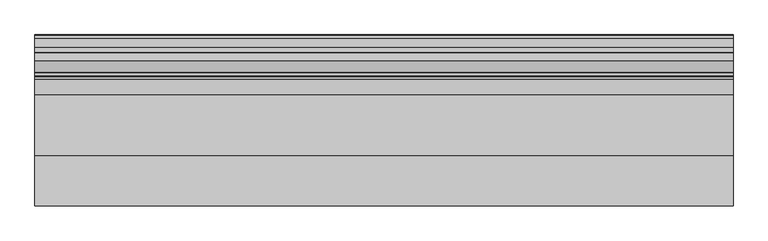
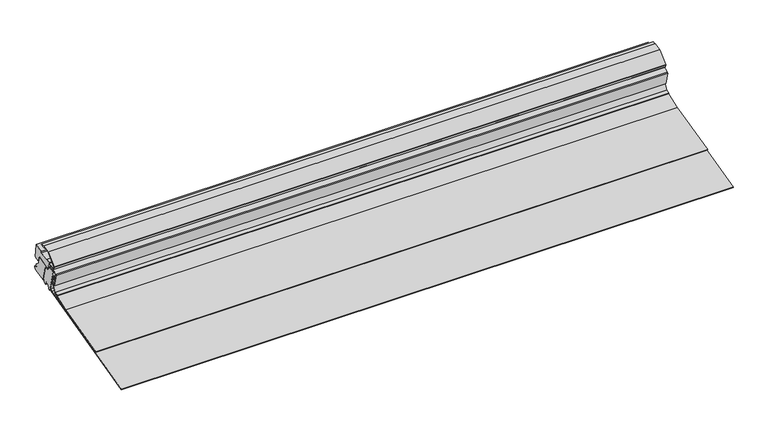
"""IFC4 building model written with IfcOpenShell, lengths in millimetres: proxy geometry, Skylight profile001 901 : Skylight profile001 901."""

from ifc_helpers import new_model, si_unit, frame, origin, place, context, project, spatial, polyline, outline, extrude, source, transform, mapped, element, save


def generic_models_6a062e64(model_context):
    return source(origin(), model_context, "Body", "SweptSolid", [
        extrude(outline(polyline([(9523.9829599, 43669.7464426), (9351.4552326, 43627.7409442), (9350.9821116, 43629.6841777), (9523.3822066, 43671.6586013), (9583.8408702, 43695.1080629), (9584.5640949, 43693.2434059), (9523.9829599, 43669.7464426)])), frame((3694.2883192, 0.0, 0.0), z_axis=(1.0, 0.0, 0.0), x_axis=(0.0, 1.0, 0.0)), (0.0, 0.0, 1.0), 2000.0),
        extrude(outline(polyline([(9598.5792608, 43722.029488), (9582.301634, 43695.3705298), (9570.3578071, 43691.0700225), (9569.6802664, 43692.9517607), (9580.9616075, 43697.0137327), (9596.4357486, 43722.3567685), (9592.5767442, 43737.7822152), (9594.516951, 43738.2675993), (9598.5792608, 43722.029488)])), frame((3694.2883192, 0.0, 0.0), z_axis=(1.0, 0.0, 0.0), x_axis=(0.0, 1.0, 0.0)), (0.0, 0.0, 1.0), 2000.0),
        extrude(outline(polyline([(9608.548635, 43692.8894811), (9604.1362045, 43685.5534517), (9206.9695462, 43585.9015861), (9206.4828193, 43587.8414565), (9602.8481566, 43687.2922651), (9606.4085244, 43693.21167), (9594.4616464, 43741.4763112), (9596.4030551, 43741.9568653), (9608.548635, 43692.8894811)])), frame((3694.2883192, 0.0, 0.0), z_axis=(1.0, 0.0, 0.0), x_axis=(0.0, 1.0, 0.0)), (0.0, 0.0, 1.0), 2000.0),
        extrude(outline(polyline([(9603.3035248, 43768.2111378), (9579.627891, 43759.3071543), (9579.0362673, 43758.1814822), (9589.836091, 43715.0117709), (9587.8958843, 43714.5263868), (9576.9108524, 43758.436423), (9578.2115618, 43760.91126), (9602.7068653, 43770.1235067), (9608.5450173, 43771.5840449), (9609.0304014, 43769.6438381), (9603.3035248, 43768.2111378)])), frame((3694.2883192, 0.0, 0.0), z_axis=(1.0, 0.0, 0.0), x_axis=(0.0, 1.0, 0.0)), (0.0, 0.0, 1.0), 2000.0),
        extrude(outline(polyline([(9645.0672166, 43810.7448228), (9644.4548349, 43815.0599326), (9622.4771809, 43810.6457496), (9590.2981236, 43779.3768871), (9590.1710895, 43777.9698492), (9591.8291283, 43771.3424198), (9593.3340619, 43770.4398277), (9615.6674335, 43776.0235989), (9616.1525398, 43774.0833227), (9593.0156633, 43768.2986598), (9590.0899861, 43770.0533507), (9588.1487662, 43777.812697), (9588.3728619, 43780.2947946), (9621.5058432, 43812.4905991), (9646.1374154, 43817.437818), (9646.7372911, 43813.2108305), (9659.5391678, 43816.3334987), (9660.0131173, 43814.3904671), (9645.0672166, 43810.7448228)])), frame((3694.2883192, 0.0, 0.0), z_axis=(1.0, 0.0, 0.0), x_axis=(0.0, 1.0, 0.0)), (0.0, 0.0, 1.0), 2000.0),
        extrude(outline(polyline([(9672.3114652, 43765.1903372), (9670.4553908, 43766.1962448), (9623.0463352, 43754.3358586), (9616.8613336, 43779.0589225), (9629.0935073, 43782.1190615), (9660.4891757, 43785.4440875), (9659.6120656, 43789.7827906), (9687.9870414, 43796.8813958), (9694.3377259, 43751.9926947), (9693.1491947, 43750.2275809), (9678.7227226, 43746.6184913), (9672.3114652, 43765.1903372)])), frame((3694.2883192, 0.0, 0.0), z_axis=(1.0, 0.0, 0.0), x_axis=(0.0, 1.0, 0.0)), (0.0, 0.0, 1.0), 2000.0),
        extrude(outline(polyline([(9689.475878, 43706.8037471), (9650.7520097, 43697.1161457), (9647.279193, 43699.1990742), (9646.7464033, 43701.3287736), (9648.5983378, 43701.7920745), (9637.0159368, 43748.0899511), (9635.1640023, 43747.6266502), (9634.6775407, 43749.5711641), (9636.7604692, 43753.0439808), (9667.7800466, 43760.8041895), (9671.2528633, 43758.7212609), (9675.7442733, 43740.9813035), (9688.175753, 43730.1920963), (9690.7976108, 43719.9252266), (9691.9552163, 43719.2309171), (9696.9023539, 43718.4778099), (9696.759928, 43715.1551973), (9691.0387865, 43707.8204765), (9689.475878, 43706.8037471)])), frame((3694.2883192, 0.0, 0.0), z_axis=(1.0, 0.0, 0.0), x_axis=(0.0, 1.0, 0.0)), (0.0, 0.0, 1.0), 2000.0),
        extrude(outline(polyline([(9632.0226951, 43701.7775274), (9619.9854477, 43698.7661533), (9618.7959335, 43686.1699212), (9612.5567495, 43684.6090563), (9604.7966767, 43715.6280904), (9603.8707473, 43715.3964494), (9592.8673693, 43759.3799855), (9614.8125618, 43764.8700434), (9617.1493935, 43755.5291179), (9623.2321013, 43750.2499166), (9632.9176503, 43752.6729632), (9634.2380448, 43747.3950021), (9637.0159368, 43748.0899511), (9648.5983378, 43701.7920745), (9643.0425537, 43700.4021767), (9644.7335843, 43693.6426868), (9634.6869888, 43691.1293168), (9632.0226951, 43701.7775274)])), frame((3694.2883192, 0.0, 0.0), z_axis=(1.0, 0.0, 0.0), x_axis=(0.0, 1.0, 0.0)), (0.0, 0.0, 1.0), 2000.0),
    ])


if __name__ == "__main__":
    model = new_model("IFC4")
    model_context = context("Model", 3, world=origin())
    ifc_project = project(units=[si_unit("LENGTHUNIT", "METRE", prefix="MILLI")], contexts=[model_context])
    site = spatial("IfcSite", under=ifc_project)
    building = spatial("IfcBuilding", under=site)
    placement = place(None, origin())
    generic_models_shape = generic_models_6a062e64(model_context)
    element("IfcBuildingElementProxy", 1, Name="Skylight profile001 901 : Skylight profile001 901", ObjectType="Skylight profile001 901 : Skylight profile001 901", at=placement, inside=building, context=model_context, shape_type="MappedRepresentation", body=[
        mapped(generic_models_shape, transform((0.0, 0.0, 0.0), x_axis=(1.0, 0.0, 0.0), y_axis=(0.0, 1.0, 0.0), z_axis=(0.0, 0.0, 1.0))),
    ])
    save(model, "model.ifc")

# Revit data of these elements
# Type "Skylight profile001 901 : Skylight profile001 901"
#   NameOverride = "Skylight profile001"
# Element 1 (IfcBuildingElementProxy, "Skylight profile001 901 : Skylight profile001 901")
#   Materials on its faces: "IfcSurfaceStyle #734"
# Materials
#   "IfcSurfaceStyle #734": class "Unassigned", colour RGB 169 181 186, transparency 0
